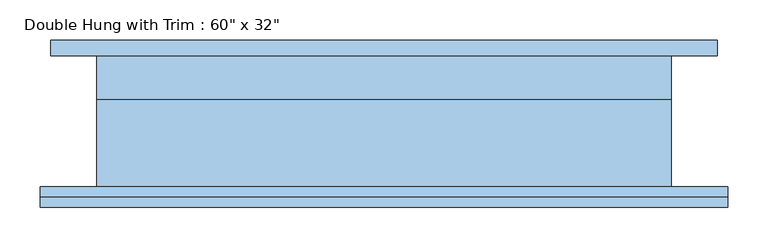
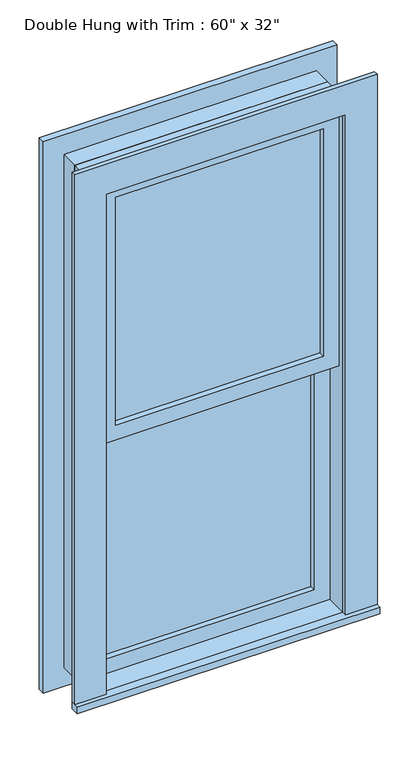
"""IFC4 building model written with IfcOpenShell, lengths in millimetres: window geometry."""

from ifc_helpers import new_model, si_unit, frame, origin, place, context, project, spatial, polyline, outline, extrude, source, transform, mapped, element, save


def window_58bf72f5(model_context):
    return source(origin(), model_context, "Body", "SweptSolid", [
        extrude(outline(polyline([(-292.1, -1.5875), (-292.1, 11.1125), (292.1, 11.1125), (292.1, -1.5875), (-292.1, -1.5875)])), frame((0.0, 0.0, 977.9), z_axis=(0.0, 0.0, 1.0), x_axis=(1.0, 0.0, 0.0)), (0.0, 0.0, 1.0), 676.275),
        extrude(outline(polyline([(1698.625, -336.55), (933.45, -336.55), (933.45, 336.55), (1698.625, 336.55), (1698.625, -336.55)]), holes=[polyline([(1654.175, -292.1), (1654.175, 292.1), (977.9, 292.1), (977.9, -292.1), (1654.175, -292.1)])]), frame((0.0, -17.4625, 0.0), z_axis=(0.0, 1.0, 0.0), x_axis=(0.0, 0.0, 1.0)), (0.0, 0.0, 1.0), 44.45),
        extrude(outline(polyline([(-425.45, -106.3625), (-425.45, -80.9625), (425.45, -80.9625), (425.45, -106.3625), (-425.45, -106.3625)])), frame((0.0, 0.0, 914.4), z_axis=(0.0, 0.0, 1.0), x_axis=(1.0, 0.0, 0.0)), (0.0, 0.0, 1.0), 19.05),
        extrude(outline(polyline([(2419.35, -336.55), (2419.35, 336.55), (933.45, 336.55), (933.45, 425.45), (2508.25, 425.45), (2508.25, -425.45), (933.45, -425.45), (933.45, -336.55), (2419.35, -336.55)])), frame((0.0, -93.6625, 0.0), z_axis=(0.0, 1.0, 0.0), x_axis=(0.0, 0.0, 1.0)), (0.0, 0.0, 1.0), 12.7),
        extrude(outline(polyline([(2495.55, 412.75), (2495.55, -412.75), (857.25, -412.75), (857.25, 412.75), (2495.55, 412.75)]), holes=[polyline([(2406.65, 323.85), (946.15, 323.85), (946.15, -323.85), (2406.65, -323.85), (2406.65, 323.85)])]), frame((0.0, 80.9625, 0.0), z_axis=(0.0, 1.0, 0.0), x_axis=(0.0, 0.0, 1.0)), (0.0, 0.0, 1.0), 19.05),
        extrude(outline(polyline([(292.1, -33.3375), (292.1, -46.0375), (-292.1, -46.0375), (-292.1, -33.3375), (292.1, -33.3375)])), frame((0.0, 0.0, 1698.625), z_axis=(0.0, 0.0, 1.0), x_axis=(1.0, 0.0, 0.0)), (0.0, 0.0, 1.0), 676.275),
        extrude(outline(polyline([(2419.35, -336.55), (1654.175, -336.55), (1654.175, 336.55), (2419.35, 336.55), (2419.35, -336.55)]), holes=[polyline([(2374.9, -292.1), (2374.9, 292.1), (1698.625, 292.1), (1698.625, -292.1), (2374.9, -292.1)])]), frame((0.0, -61.9125, 0.0), z_axis=(0.0, 1.0, 0.0), x_axis=(0.0, 0.0, 1.0)), (0.0, 0.0, 1.0), 44.45),
        extrude(outline(polyline([(2438.4, -355.6), (914.4, -355.6), (914.4, 355.6), (2438.4, 355.6), (2438.4, -355.6)]), holes=[polyline([(2406.65, -323.85), (2406.65, 323.85), (946.15, 323.85), (946.15, -323.85), (2406.65, -323.85)])]), frame((0.0, 26.9875, 0.0), z_axis=(0.0, 1.0, 0.0), x_axis=(0.0, 0.0, 1.0)), (0.0, 0.0, 1.0), 53.975),
        extrude(outline(polyline([(2438.4, 355.6), (2438.4, -355.6), (914.4, -355.6), (914.4, 355.6), (2438.4, 355.6)]), holes=[polyline([(2419.35, 336.55), (933.45, 336.55), (933.45, -336.55), (2419.35, -336.55), (2419.35, 336.55)])]), frame((0.0, -80.9625, 0.0), z_axis=(0.0, 1.0, 0.0), x_axis=(0.0, 0.0, 1.0)), (0.0, 0.0, 1.0), 107.95),
    ])


if __name__ == "__main__":
    model = new_model("IFC4")
    model_context = context("Model", 3, world=origin())
    ifc_project = project(units=[si_unit("LENGTHUNIT", "METRE", prefix="MILLI")], contexts=[model_context])
    site = spatial("IfcSite", under=ifc_project)
    building = spatial("IfcBuilding", under=site)
    placement = place(None, origin())
    window_shape = window_58bf72f5(model_context)
    element("IfcWindow", 1, ObjectType="Double Hung with Trim : 60\" x 32\"", at=placement, inside=building, context=model_context, shape_type="MappedRepresentation", body=[
        mapped(window_shape, transform((0.0, 0.0, 0.0), x_axis=(1.0, 0.0, 0.0), y_axis=(0.0, 1.0, 0.0), z_axis=(0.0, 0.0, 1.0))),
    ])
    save(model, "model.ifc")

# Revit data of these elements
# Type "Double Hung with Trim : 60\" x 32\""
#   Type Mark = "62"
#   COBie.Type.CreatedBy = "doug.wood@us.ibm.com"
#   COBie.Type.CreatedOn = "2016-04-14T02:07:26"
#   COBie.Type.Name = "Windows_Double Hung with Trim_60\" x 32\"_62"
#   COBie.Type.Category = "23-30 20 17 17 14 : Double-Hung Windows"
#   COBie.Type.Description = "Double Hung with Trim_60\" x 32\""
#   COBie.Type.Manufacturer = ""
#   COBie.Type.ModelNumber = ""
#   Construction Type Id = "GSP4R"
#   Assembly Code = "B2020100"
#   Analytic Construction = "1/8 in Pilkington single glazing"
#   COBie.Type.ReplacementCost = 0
#   Visual Light Transmittance = 0.9
#   Solar Heat Gain Coefficient = 0.78
#   Heat Transfer Coefficient (U) = 3.6886 W/(m²·K)
#   Height = 5' - 0"
#   Default Sill Height = 3' - 0"
#   Trim Projection - Ext. = 0' - 0 1/2"
#   Trim Projection - Int. = 0' - 0 3/4"
#   Trim Width - Exterior = 0' - 3 1/2"
#   Trim Width - Interior = 0' - 3 1/2"
#   Width = 2' - 4"
#   Window Inset = 0' - 0 3/4"
#   COBie.Type = no
#   Glass Pane Material = Glass
#   Sash Material = Sash - White
#   Trim Exterior Material = Trim - White
#   Trim Interior Material = Trim - White
#   Wall Closure = (empty or 0)
# Element 1 (IfcWindow, "Double Hung with Trim : 60\" x 32\"")
#   Materials on its faces: "Sash - White", "Trim - White", "Glass"
# Materials
#   "Glass": class "Glass", colour RGB 0 128 192, transparency 0.75, Description = "Soda Lime Glass", Cost = 0
#   "Sash - White": class "Wood", colour RGB 255 255 255, transparency 0, Cost = 0
#   "Trim - White": class "Wood", colour RGB 255 255 255, transparency 0, Cost = 0
